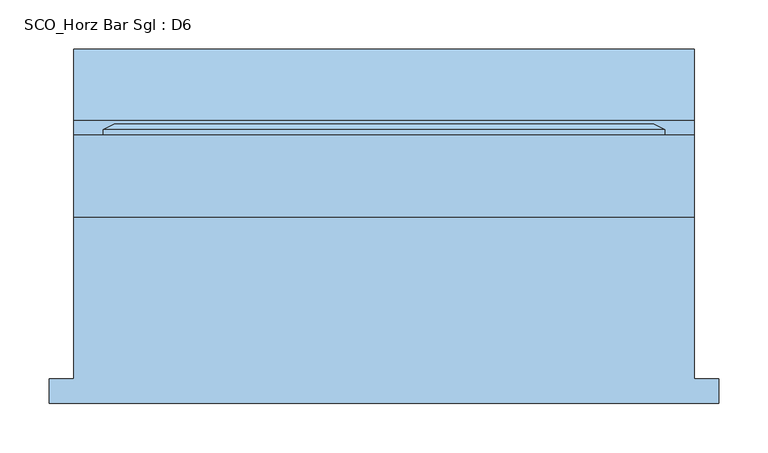
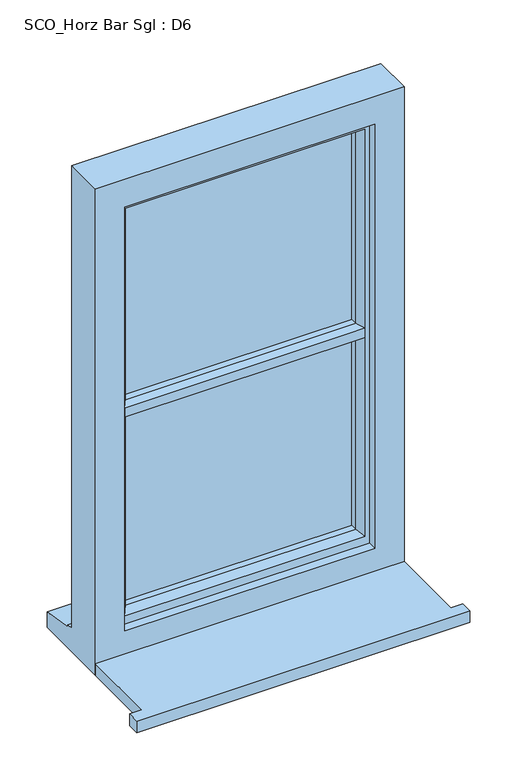
"""IFC4 building model written with IfcOpenShell, lengths in millimetres: window geometry, SCO_Horz Bar Sgl : D6."""

from ifc_helpers import new_model, si_unit, frame, origin, place, context, project, spatial, polyline, outline, extrude, faceted_brep, source, transform, mapped, element, save


def sco_horz_bar_sgl_d6_79d9ea54(model_context):
    return source(origin(), model_context, "Body", "SolidModel", [
        extrude(outline(polyline([(-340.0, -191.5434322), (-340.0, -166.5434322), (-315.0, -166.5434322), (-315.0, -2.0434322), (315.0, -2.0434322), (315.0, -166.5434322), (340.0, -166.5434322), (340.0, -191.5434322), (-340.0, -191.5434322)])), frame((0.0, 0.0, 1060.0), z_axis=(0.0, 0.0, 1.0), x_axis=(1.0, 0.0, 0.0)), (0.0, 0.0, 1.0), 25.0),
        faceted_brep([(-315.0, -2.0434322, 1060.0), (315.0, -2.0434322, 1060.0), (315.0, -2.0434322, 2110.0), (-315.0, -2.0434322, 2110.0), (-255.0, -2.0434322, 2050.0), (255.0, -2.0434322, 2050.0), (255.0, -2.0434322, 1135.0), (-255.0, -2.0434322, 1135.0), (-315.0, 80.9565678, 2110.0), (-315.0, 80.9565678, 1111.0), (-315.0, 95.9565678, 1109.68767), (-315.0, 95.9565678, 1104.7449676), (-315.0, 168.4565678, 1093.8088847), (-315.0, 168.4565678, 1060.0), (315.0, 80.9565678, 2110.0), (315.0, 80.9565678, 1111.0), (-275.0, 80.9565678, 2070.0), (-275.0, 80.9565678, 1123.0), (275.0, 80.9565678, 1123.0), (275.0, 80.9565678, 2070.0), (-275.0, 15.9565678, 2070.0), (-275.0, 15.9565678, 1123.0), (275.0, 15.9565678, 2070.0), (275.0, 15.9565678, 1123.0), (-255.0, 15.9565678, 2050.0), (-255.0, 15.9565678, 1135.0), (255.0, 15.9565678, 1135.0), (255.0, 15.9565678, 2050.0), (315.0, 168.4565678, 1060.0), (315.0, 168.4565678, 1093.8088847), (315.0, 95.9565678, 1104.7449676), (315.0, 95.9565678, 1109.68767)], [[[0, 1, 2, 3], [4, 5, 6, 7]], [[0, 3, 8, 9, 10, 11, 12, 13]], [[9, 8, 14, 15], [16, 17, 18, 19]], [[17, 16, 20, 21]], [[20, 22, 23, 21], [24, 25, 26, 27]], [[24, 4, 7, 25]], [[3, 2, 14, 8]], [[16, 19, 22, 20]], [[5, 4, 24, 27]], [[15, 14, 2, 1, 28, 29, 30, 31]], [[19, 18, 23, 22]], [[5, 27, 26, 6]], [[28, 1, 0, 13]], [[29, 28, 13, 12]], [[30, 29, 12, 11]], [[31, 30, 11, 10]], [[15, 31, 10, 9]], [[21, 23, 18, 17]], [[7, 6, 26, 25]]]),
        extrude(outline(polyline([(245.1480377, 44.9565678), (-245.0, 44.9565678), (-245.0, 68.9565678), (245.1480377, 68.9565678), (245.1480377, 44.9565678)])), frame((0.0, 0.0, 1153.0), z_axis=(0.0, 0.0, 1.0), x_axis=(1.0, 0.0, 0.0)), (0.0, 0.0, 1.0), 434.3307627),
        extrude(outline(polyline([(245.1480377, 44.9565678), (-245.0, 44.9565678), (-245.0, 68.9565678), (245.1480377, 68.9565678), (245.1480377, 44.9565678)])), frame((0.0, 0.0, 1597.6692373), z_axis=(0.0, 0.0, 1.0), x_axis=(1.0, 0.0, 0.0)), (0.0, 0.0, 1.0), 442.3307627),
        extrude(outline(polyline([(92.5035732, 1597.6692373), (92.5035732, 1587.3307627), (86.8277797, 1577.5), (68.9565678, 1577.5), (68.9565678, 1584.5), (44.9565678, 1584.5), (44.9565678, 1577.5), (30.4494677, 1577.5), (15.9565678, 1582.6480377), (15.9565678, 1602.3519623), (30.4494677, 1607.5), (44.9565678, 1607.5), (44.9565678, 1600.5), (68.9565678, 1600.5), (68.9565678, 1607.5), (86.8277797, 1607.5), (92.5035732, 1597.6692373)])), frame((-245.1480377, 0.0, 0.0), z_axis=(1.0, 0.0, 0.0), x_axis=(0.0, 1.0, 0.0)), (0.0, 0.0, 1.0), 490.2960754),
        faceted_brep([(-285.0, 80.9565678, 2072.0), (-285.0, 86.7300705, 2072.0), (-285.0, 86.7300705, 1113.0), (-285.0, 80.9565678, 1113.0), (-275.0, 15.9565678, 2062.0), (-275.0, 80.9565678, 2062.0), (-275.0, 80.9565678, 1123.0), (-275.0, 15.9565678, 1123.0), (-235.0, 30.4494677, 2022.0), (-245.1480377, 15.9565678, 2032.1480377), (-245.1480377, 15.9565678, 1152.8519623), (-235.0, 30.4494677, 1163.0), (-235.0, 44.9565678, 2022.0), (-235.0, 44.9565678, 1163.0), (-245.0, 68.9565678, 2032.0), (-245.0, 44.9565678, 2032.0), (-245.0, 44.9565678, 1153.0), (-245.0, 68.9565678, 1153.0), (-235.0, 86.7300705, 2022.0), (-235.0, 68.9565678, 2022.0), (-235.0, 68.9565678, 1163.0), (-235.0, 86.7300705, 1163.0), (-245.0, 92.5035732, 2032.0), (-245.0, 92.5035732, 1153.0), (-274.2153903, 92.5035732, 2061.2153903), (-274.2153903, 92.5035732, 1123.7846097), (285.0, 86.7300705, 1113.0), (285.0, 80.9565678, 1113.0), (275.0, 80.9565678, 1123.0), (275.0, 15.9565678, 1123.0), (245.1480377, 15.9565678, 1152.8519623), (235.0, 30.4494677, 1163.0), (235.0, 44.9565678, 1163.0), (245.0, 44.9565678, 1153.0), (245.0, 68.9565678, 1153.0), (235.0, 68.9565678, 1163.0), (235.0, 86.7300705, 1163.0), (245.0, 92.5035732, 1153.0), (274.2153903, 92.5035732, 1123.7846097), (285.0, 86.7300705, 2072.0), (285.0, 80.9565678, 2072.0), (275.0, 80.9565678, 2062.0), (275.0, 15.9565678, 2062.0), (245.1480377, 15.9565678, 2032.1480377), (235.0, 30.4494677, 2022.0), (235.0, 44.9565678, 2022.0), (245.0, 44.9565678, 2032.0), (245.0, 68.9565678, 2032.0), (235.0, 68.9565678, 2022.0), (235.0, 86.7300705, 2022.0), (245.0, 92.5035732, 2032.0), (274.2153903, 92.5035732, 2061.2153903)], [[[0, 1, 2, 3]], [[4, 5, 6, 7]], [[8, 9, 10, 11]], [[12, 8, 11, 13]], [[14, 15, 16, 17]], [[18, 19, 20, 21]], [[22, 18, 21, 23]], [[1, 24, 25, 2]], [[3, 2, 26, 27]], [[7, 6, 28, 29]], [[11, 10, 30, 31]], [[13, 11, 31, 32]], [[17, 16, 33, 34]], [[21, 20, 35, 36]], [[23, 21, 36, 37]], [[2, 25, 38, 26]], [[27, 26, 39, 40]], [[29, 28, 41, 42]], [[31, 30, 43, 44]], [[32, 31, 44, 45]], [[34, 33, 46, 47]], [[36, 35, 48, 49]], [[37, 36, 49, 50]], [[26, 38, 51, 39]], [[40, 39, 1, 0]], [[3, 27, 40, 0], [5, 41, 28, 6]], [[42, 41, 5, 4]], [[7, 29, 42, 4], [9, 43, 30, 10]], [[44, 43, 9, 8]], [[45, 44, 8, 12]], [[15, 46, 33, 16], [13, 32, 45, 12]], [[47, 46, 15, 14]], [[17, 34, 47, 14], [19, 48, 35, 20]], [[49, 48, 19, 18]], [[50, 49, 18, 22]], [[24, 51, 38, 25], [23, 37, 50, 22]], [[39, 51, 24, 1]]]),
    ])


if __name__ == "__main__":
    model = new_model("IFC4")
    model_context = context("Model", 3, world=origin())
    ifc_project = project(units=[si_unit("LENGTHUNIT", "METRE", prefix="MILLI")], contexts=[model_context])
    site = spatial("IfcSite", under=ifc_project)
    building = spatial("IfcBuilding", under=site)
    placement = place(None, origin())
    sco_horz_bar_sgl_d6_shape = sco_horz_bar_sgl_d6_79d9ea54(model_context)
    element("IfcWindow", 1, ObjectType="SCO_Horz Bar Sgl : D6", at=placement, inside=building, context=model_context, shape_type="MappedRepresentation", body=[
        mapped(sco_horz_bar_sgl_d6_shape, transform((0.0, 0.0, 0.0), x_axis=(1.0, 0.0, 0.0), y_axis=(0.0, 1.0, 0.0), z_axis=(0.0, 0.0, 1.0))),
    ])
    save(model, "model.ifc")

# Revit data of these elements
# Type "SCO_Horz Bar Sgl : D6"
#   Type Mark = "W6"
#   Operation = "SinglePanel"
#   Manufacturer = "Revit"
#   Keynote = "L10"
#   Wrap Layers (Ext) from Ext = 102.5 mm
#   Wrap Layers (Int) from Ext = 177.5 mm
#   Window Board Projection = 25 mm
#   Window Board Extension = 25 mm
#   Rough Width = 630 mm
#   Rough Height = 1050 mm
#   Height = 1050 mm
#   Width = 630 mm
#   Glazing Thickness = 24 mm
#   FrameOffset - External = 102.5 mm
#   Frame Depth = 65 mm
#   Ext Leaf Thickness (Scot) = 102.5 mm
#   Ext Leaf Overlap (Scot) = 25 mm
#   Default Head Height = 2110 mm
#   Cill Depth = 87.5 mm
#   Cavity Closer Width = 50 mm
#   Cavity Closer Offset from Ext = 102.5 mm
#   Cavity Closer Depth = 85 mm
#   Vis - Cavity Closers = yes
#   Material Trim = Window Frame
#   Material Glass = Glass
#   Material Frame = Window Frame
#   Wall Closure = (empty or 0)
# Element 1 (IfcWindow, "SCO_Horz Bar Sgl : D6")
#   Materials on its faces: "Window Frame", "Glass"
# Materials
#   "Window Frame": class "Miscellaneous", colour RGB 249 249 249, transparency 0
#   "Glass": class "Glass", colour RGB 0 128 192, transparency 0.75
